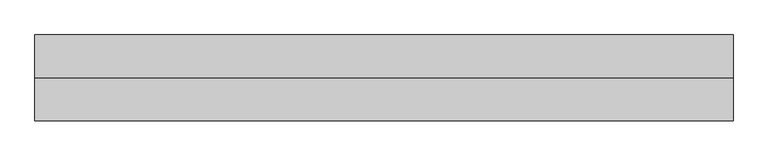
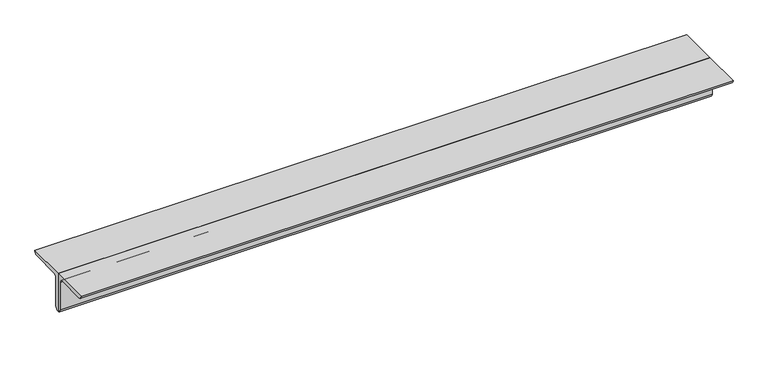
"""IFC4 building model written with IfcOpenShell, lengths in millimetres: member geometry, 0123_Steel Framing_2Ls-KSD3502 : H_SB_AR_S04_2Ls-130x130x12_VBR1."""

from ifc_helpers import new_model, si_unit, point, frame, frame_2d, origin, place, context, project, spatial, polyline, circle_curve, trimmed, segment, composite_curve, outline, extrude, source, transform, mapped, element, save


def member_893a5a9c(model_context):
    return source(origin(), model_context, "Body", "SweptSolid", [
        extrude(outline(composite_curve([segment(polyline([(0.0, 36.4), (130.0, 36.4)]), True, "CONTINUOUS"), segment(trimmed(circle_curve(frame_2d((118.0, 36.4)), 12.0), [point((130.0, 36.4))], [point((118.0, 24.4))], False, "CARTESIAN"), True, "CONTINUOUS"), segment(polyline([(118.0, 24.4), (24.0, 24.4)]), True, "CONTINUOUS"), segment(trimmed(circle_curve(frame_2d((24.0, 12.4)), 12.0), [point((24.0, 24.4))], [point((12.0, 12.4))], True, "CARTESIAN"), True, "CONTINUOUS"), segment(polyline([(12.0, 12.4), (12.0, -81.6)]), True, "CONTINUOUS"), segment(trimmed(circle_curve(frame_2d((0.0, -81.6)), 12.0), [point((12.0, -81.6))], [point((0.0, -93.6))], False, "CARTESIAN"), True, "CONTINUOUS"), segment(polyline([(0.0, -93.6), (0.0, 36.4)]), True, "CONTINUOUS")], self_intersect=False)), frame((-991.4315887, 0.0, 0.0), z_axis=(1.0, 0.0, 0.0), x_axis=(0.0, 1.0, 0.0)), (0.0, 0.0, 1.0), 2118.004285),
        extrude(outline(composite_curve([segment(polyline([(0.0, 36.4), (0.0, -93.6)]), True, "CONTINUOUS"), segment(trimmed(circle_curve(frame_2d((0.0, -81.6)), 12.0), [point((0.0, -93.6))], [point((-12.0, -81.6))], False, "CARTESIAN"), True, "CONTINUOUS"), segment(polyline([(-12.0, -81.6), (-12.0, 12.4)]), True, "CONTINUOUS"), segment(trimmed(circle_curve(frame_2d((-24.0, 12.4)), 12.0), [point((-12.0, 12.4))], [point((-24.0, 24.4))], True, "CARTESIAN"), True, "CONTINUOUS"), segment(polyline([(-24.0, 24.4), (-118.0, 24.4)]), True, "CONTINUOUS"), segment(trimmed(circle_curve(frame_2d((-118.0, 36.4)), 12.0), [point((-118.0, 24.4))], [point((-130.0, 36.4))], False, "CARTESIAN"), True, "CONTINUOUS"), segment(polyline([(-130.0, 36.4), (0.0, 36.4)]), True, "CONTINUOUS")], self_intersect=False)), frame((-991.4315887, 0.0, 0.0), z_axis=(1.0, 0.0, 0.0), x_axis=(0.0, 1.0, 0.0)), (0.0, 0.0, 1.0), 2118.004285),
    ])


if __name__ == "__main__":
    model = new_model("IFC4")
    model_context = context("Model", 3, world=origin())
    ifc_project = project(units=[si_unit("LENGTHUNIT", "METRE", prefix="MILLI")], contexts=[model_context])
    site = spatial("IfcSite", under=ifc_project)
    building = spatial("IfcBuilding", under=site)
    placement = place(None, origin())
    member_shape = member_893a5a9c(model_context)
    element("IfcMember", 1, ObjectType="0123_Steel Framing_2Ls-KSD3502 : H_SB_AR_S04_2Ls-130x130x12_VBR1", at=placement, inside=building, context=model_context, shape_type="MappedRepresentation", body=[
        mapped(member_shape, transform((0.0, 0.0, 0.0), x_axis=(1.0, 0.0, 0.0), y_axis=(0.0, 1.0, 0.0), z_axis=(0.0, 0.0, 1.0))),
    ])
    save(model, "model.ifc")

# Revit data of these elements
# Type "0123_Steel Framing_2Ls-KSD3502 : H_SB_AR_S04_2Ls-130x130x12_VBR1"
#   Assembly Code = "B10"
#   Legs = "SLBB"
#   W = 8.97
#   Perimeter = 1.04 m²/m
#   Nominal Weight = 46.80 kgf/m
#   Length [instance default] = 1000 mm
#   Space = 0 mm
#   b = 130 mm
#   d = 130 mm
#   t = 12 mm
#   y = 36.4 mm
#   A = 0.005952 m²
#   Structural Material [instance default] = Steel ASTM A36
# Element 1 (IfcMember, "0123_Steel Framing_2Ls-KSD3502 : H_SB_AR_S04_2Ls-130x130x12_VBR1")
#   Structural Material = Steel, 45-345
#   Materials on its faces: "Steel, 45-345"
# Materials
#   "Steel ASTM A36": class "Metal", colour RGB 199 199 199, transparency 0, Description = "Structural steel, ASTM A36 Grade B, mill finish", Cost = 0
#   "Steel, 45-345": class "Metal", colour RGB 189 187 185, transparency 0, Description = "Steel 345 MPa", Cost = 0
